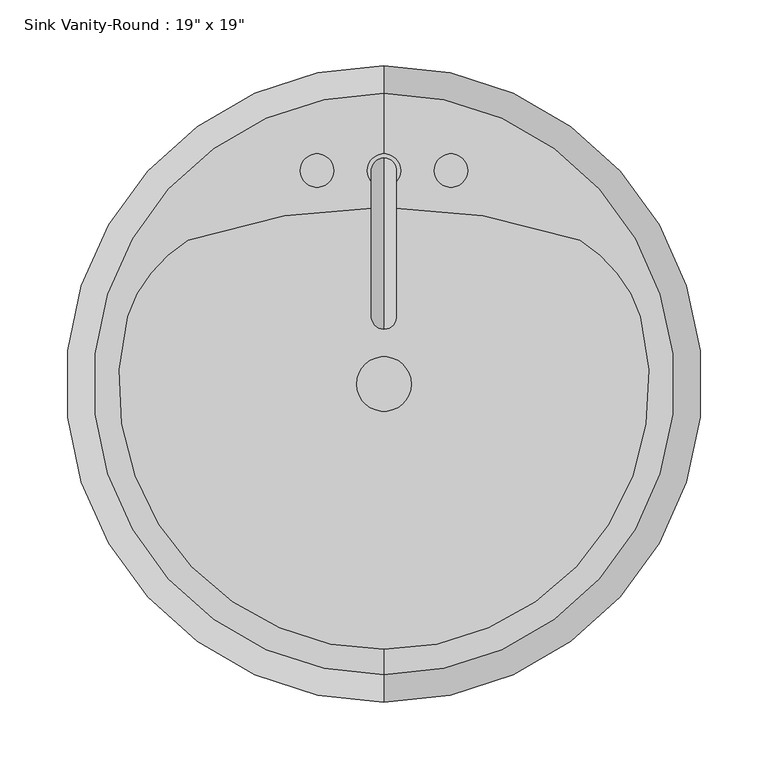
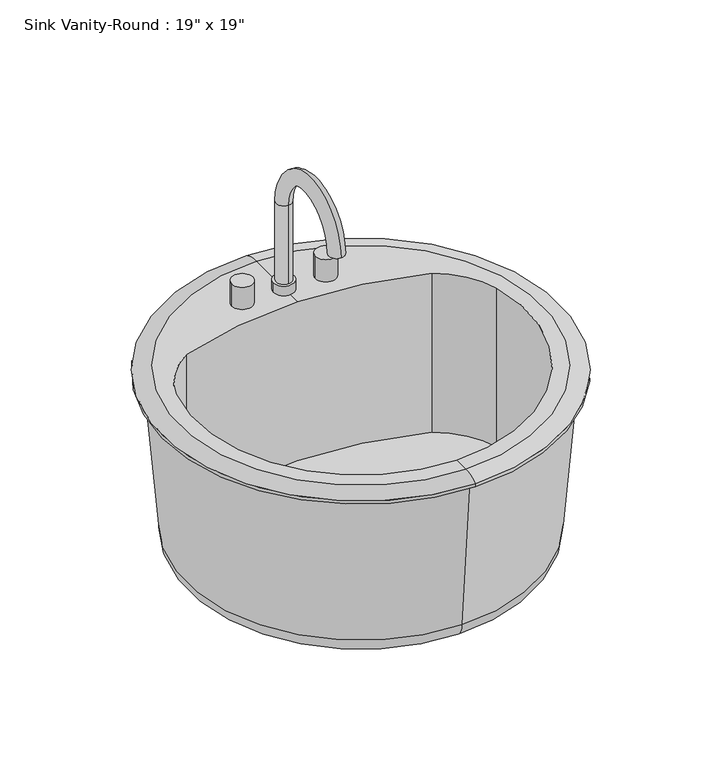
"""IFC4 building model written with IfcOpenShell, lengths in millimetres: flow terminal geometry."""

import ifcopenshell
import ifcopenshell.guid

model = None  # the IFC model being written
_history = None  # IfcOwnerHistory: only IFC2X3 demands one
_inside = {}  # id of a spatial element -> (the spatial element, [elements in it])
_under = {}  # id of a project, library or spatial element -> (it, [spatial elements below it])
_declared = {}  # id of a project -> (the project, [libraries it declares])
_typed = {}  # id of a type object -> (the type object, [elements of that type])
_made_of = {}  # id of a material, layer set ... -> (it, [elements and type objects made of it])


def new_model(schema):
    """Start an empty IFC model of exactly this schema.

    Asked for "IFC4X3", IfcOpenShell would pick the latest addendum, in which some entities
    have other attributes; the version numbers below select the first issue.
    IFC2X3 requires an IfcOwnerHistory on every rooted entity: one is made here for all.
    """
    global model, _history
    if schema == "IFC4X3":
        model = ifcopenshell.file(schema_version=(4, 3, 0, 0))
    else:
        model = ifcopenshell.file(schema=schema)
    _inside.clear()
    _under.clear()
    _declared.clear()
    _typed.clear()
    _made_of.clear()
    _history = None
    if model.schema == "IFC2X3":
        org = make("IfcOrganization", Name="unknown")
        user = make(
            "IfcPersonAndOrganization",
            ThePerson=make("IfcPerson", FamilyName="unknown"),
            TheOrganization=org,
        )
        app = make(
            "IfcApplication",
            ApplicationDeveloper=org,
            Version="unknown",
            ApplicationFullName="unknown",
            ApplicationIdentifier="unknown",
        )
        _history = make(
            "IfcOwnerHistory",
            OwningUser=user,
            OwningApplication=app,
            ChangeAction="ADDED",
            CreationDate=0,
        )
    return model


def make(cls, **values):
    """One entity of the class cls with the attributes given. An attribute that is None is left unset."""
    return model.create_entity(
        cls, **{name: value for name, value in values.items() if value is not None}
    )


def rooted(cls, **values):
    """An entity with a GlobalId (a new one), such as an element, a storey or a relation."""
    return make(cls, GlobalId=ifcopenshell.guid.new(), OwnerHistory=_history, **values)


def si_unit(unit_type, name, prefix=None):
    """IfcSIUnit, for example si_unit("LENGTHUNIT", "METRE", prefix="MILLI")."""
    return make("IfcSIUnit", UnitType=unit_type, Prefix=prefix, Name=name)


def assignment(units):
    """IfcUnitAssignment: the units of a project."""
    return None if units is None else make("IfcUnitAssignment", Units=units)


def point(xyz):
    """IfcCartesianPoint."""
    return None if xyz is None else make("IfcCartesianPoint", Coordinates=xyz)


def direction(xyz):
    """IfcDirection."""
    return None if xyz is None else make("IfcDirection", DirectionRatios=xyz)


def frame(location, z_axis=None, x_axis=None):
    """IfcAxis2Placement3D, a coordinate frame: its origin and axes. An axis left out is left unset."""
    return make(
        "IfcAxis2Placement3D",
        Location=point(location),
        Axis=direction(z_axis),
        RefDirection=direction(x_axis),
    )


def frame_2d(location, x_axis=None):
    """IfcAxis2Placement2D, a coordinate frame in the plane: its origin and x axis."""
    return make(
        "IfcAxis2Placement2D", Location=point(location), RefDirection=direction(x_axis)
    )


def origin():
    """The frame at (0, 0, 0) with its axes left unset."""
    return frame((0.0, 0.0, 0.0))


def place(relative_to, where):
    """IfcLocalPlacement: puts the frame where relative to a parent placement (None: the world)."""
    return make(
        "IfcLocalPlacement", PlacementRelTo=relative_to, RelativePlacement=where
    )


def context(
    kind, dimensions, precision=None, world=None, true_north=None, identifier=None
):
    """IfcGeometricRepresentationContext, for example the 3D "Model" context."""
    return make(
        "IfcGeometricRepresentationContext",
        ContextIdentifier=identifier,
        ContextType=kind,
        CoordinateSpaceDimension=dimensions,
        Precision=precision,
        WorldCoordinateSystem=world,
        TrueNorth=true_north,
    )


def project(units=None, contexts=None):
    """IfcProject with its units and contexts."""
    return rooted(
        "IfcProject",
        Name="project",
        RepresentationContexts=contexts,
        UnitsInContext=assignment(units),
    )


def spatial(cls, under=None, at=None, **own):
    """A site, building, storey or space (cls), placed at a placement, below another one or the project."""
    s = rooted(cls, ObjectPlacement=at, **own)
    if under is not None:
        _under.setdefault(under.id(), (under, []))[1].append(s)
    return s


def polyline(points):
    """IfcPolyline through the points."""
    return make("IfcPolyline", Points=[point(p) for p in points])


def circle_curve(where, radius):
    """IfcCircle in the frame where."""
    return make("IfcCircle", Position=where, Radius=radius)


def ellipse_curve(where, semi_axis1, semi_axis2):
    """IfcEllipse in the frame where."""
    return make(
        "IfcEllipse", Position=where, SemiAxis1=semi_axis1, SemiAxis2=semi_axis2
    )


def trimmed(basis, trim1, trim2, sense, master):
    """IfcTrimmedCurve: the piece of a basis curve between two trims."""
    return make(
        "IfcTrimmedCurve",
        BasisCurve=basis,
        Trim1=trim1,
        Trim2=trim2,
        SenseAgreement=sense,
        MasterRepresentation=master,
    )


def segment(curve, same_sense, transition):
    """IfcCompositeCurveSegment."""
    return make(
        "IfcCompositeCurveSegment",
        Transition=transition,
        SameSense=same_sense,
        ParentCurve=curve,
    )


def composite_curve(segments, self_intersect=None):
    """IfcCompositeCurve: segments joined end to end."""
    return make("IfcCompositeCurve", Segments=segments, SelfIntersect=self_intersect)


def outline(outer, holes=None, kind="AREA"):
    """IfcArbitraryClosedProfileDef: a profile drawn as a closed curve; with holes, ...WithVoids."""
    if holes is None:
        return make("IfcArbitraryClosedProfileDef", ProfileType=kind, OuterCurve=outer)
    return make(
        "IfcArbitraryProfileDefWithVoids",
        ProfileType=kind,
        OuterCurve=outer,
        InnerCurves=holes,
    )


def extrude(swept, where, along, depth):
    """IfcExtrudedAreaSolid: the profile swept, set in the frame where, extruded along a direction by depth."""
    return make(
        "IfcExtrudedAreaSolid",
        SweptArea=swept,
        Position=where,
        ExtrudedDirection=direction(along),
        Depth=depth,
    )


def shape(context_of_items, identifier, shape_type, items):
    """IfcShapeRepresentation: the items that make up one representation, for example the "Body"."""
    return make(
        "IfcShapeRepresentation",
        ContextOfItems=context_of_items,
        RepresentationIdentifier=identifier,
        RepresentationType=shape_type,
        Items=items,
    )


def source(mapping_origin, context_of_items, identifier, shape_type, items):
    """IfcRepresentationMap: a shape defined once, which mapped items show again and again."""
    return make(
        "IfcRepresentationMap",
        MappingOrigin=mapping_origin,
        MappedRepresentation=shape(context_of_items, identifier, shape_type, items),
    )


def transform(
    local_origin,
    x_axis=None,
    y_axis=None,
    z_axis=None,
    scale=None,
    scale2=None,
    scale3=None,
    uniform=True,
):
    """IfcCartesianTransformationOperator3D, or its non-uniform kind. x_axis, y_axis, z_axis: its Axis1, 2, 3."""
    if uniform:
        return make(
            "IfcCartesianTransformationOperator3D",
            Axis1=direction(x_axis),
            Axis2=direction(y_axis),
            LocalOrigin=point(local_origin),
            Scale=scale,
            Axis3=direction(z_axis),
        )
    return make(
        "IfcCartesianTransformationOperator3DnonUniform",
        Axis1=direction(x_axis),
        Axis2=direction(y_axis),
        LocalOrigin=point(local_origin),
        Scale=scale,
        Axis3=direction(z_axis),
        Scale2=scale2,
        Scale3=scale3,
    )


def mapped(mapping_source, mapping_target):
    """IfcMappedItem: shows the shape of a source again, moved by a transform."""
    return make(
        "IfcMappedItem", MappingSource=mapping_source, MappingTarget=mapping_target
    )


def made_of(thing, what):
    """Note that an element or type object is made of a material, layer set ...; save() writes the relation."""
    if what is not None:
        _made_of.setdefault(what.id(), (what, []))[1].append(thing)
    return thing


def element(
    cls,
    number,
    at=None,
    inside=None,
    cuts=None,
    type_object=None,
    material=None,
    context=None,
    identifier="Body",
    shape_type=None,
    held_by="IfcProductDefinitionShape",
    body=None,
    shapes=None,
    **own,
):
    """One element of the class cls, such as IfcWall. Its Tag is "e" and its number.

    at: its placement. inside: the storey or other place that contains it. cuts: it is an
    opening in that element (IfcRelVoidsElement). A single representation is given by context,
    identifier, shape_type and body (its items); several are given by shapes. held_by: the class
    of the entity that holds the representations. save() writes the other relations.
    """
    e = rooted(cls, Tag="e%d" % number, ObjectPlacement=at, **own)
    if body is not None:
        shapes = [shape(context, identifier, shape_type, body)]
    if shapes is not None:
        e.Representation = make(held_by, Representations=shapes)
    if inside is not None:
        _inside.setdefault(inside.id(), (inside, []))[1].append(e)
    if cuts is not None:
        rooted(
            "IfcRelVoidsElement", RelatingBuildingElement=cuts, RelatedOpeningElement=e
        )
    if type_object is not None:
        _typed.setdefault(type_object.id(), (type_object, []))[1].append(e)
    return made_of(e, material)


def aggregate(whole, parts):
    """IfcRelAggregates: a whole, such as a stair, and the parts it consists of."""
    return rooted("IfcRelAggregates", RelatingObject=whole, RelatedObjects=parts)


def save(model, path):
    """Write the relations noted so far, then the file.

    IfcRelAggregates (storeys below a building ...), IfcRelContainedInSpatialStructure (elements
    in a storey), IfcRelDefinesByType, IfcRelAssociatesMaterial and IfcRelDeclares: one each for
    every whole, place, type object, material and project.
    """
    for whole, parts in _under.values():
        aggregate(whole, parts)
    for where, things in _inside.values():
        rooted(
            "IfcRelContainedInSpatialStructure",
            RelatedElements=things,
            RelatingStructure=where,
        )
    for kind, things in _typed.values():
        rooted("IfcRelDefinesByType", RelatedObjects=things, RelatingType=kind)
    for what, things in _made_of.values():
        rooted("IfcRelAssociatesMaterial", RelatedObjects=things, RelatingMaterial=what)
    for by, libraries in _declared.values():
        rooted("IfcRelDeclares", RelatingContext=by, RelatedDefinitions=libraries)
    model.write(path)


def plane_surface(at):
    """IfcPlane: the flat surface through the origin of the frame at, square to its z axis."""
    return make("IfcPlane", Position=at)


def cylinder_surface(at, radius):
    """IfcCylindricalSurface: all points at the distance radius from the z axis of the frame at."""
    return make("IfcCylindricalSurface", Position=at, Radius=radius)


def revolved_surface(curve, axis_point, axis_direction):
    """IfcSurfaceOfRevolution: the curve turned about the line through axis_point along axis_direction."""
    return make(
        "IfcSurfaceOfRevolution",
        SweptCurve=make("IfcArbitraryOpenProfileDef", ProfileType="CURVE", Curve=curve),
        AxisPosition=make("IfcAxis1Placement", Location=point(axis_point), Axis=direction(axis_direction)),
    )


def advanced_brep(points, edges, surfaces, faces):
    """IfcAdvancedBrep: a solid bounded by faces that lie on surfaces and meet in shared edges.

    An edge is (start, end): straight between two places in points (the first is 0);
    or (start, end, curve); or (start, end, curve, False) where it runs against its curve.
    A face is (place in surfaces, loops), or (place, loops, False) where it looks against
    its surface's normal. A loop lists edges by number (the first is 1), with a minus sign
    where the edge is run from its end to its start. The first loop is the outer one.
    """
    corners = [point(p) for p in points]
    vertices = [make("IfcVertexPoint", VertexGeometry=c) for c in corners]
    made = []
    for start, end, *more in edges:
        made.append(
            make(
                "IfcEdgeCurve",
                EdgeStart=vertices[start],
                EdgeEnd=vertices[end],
                EdgeGeometry=more[0] if more else make("IfcPolyline", Points=[corners[start], corners[end]]),
                SameSense=more[1] if len(more) > 1 else True,
            )
        )
    hull = []
    for where, loops, *sense in faces:
        bounds = []
        for j, loop in enumerate(loops):
            ring = [make("IfcOrientedEdge", EdgeElement=made[abs(k) - 1], Orientation=k > 0) for k in loop]
            bounds.append(
                make(
                    "IfcFaceOuterBound" if j == 0 else "IfcFaceBound",
                    Bound=make("IfcEdgeLoop", EdgeList=ring),
                    Orientation=True,
                )
            )
        hull.append(make("IfcAdvancedFace", Bounds=bounds, FaceSurface=surfaces[where], SameSense=sense[0] if sense else True))
    return make("IfcAdvancedBrep", Outer=make("IfcClosedShell", CfsFaces=hull))


def flow_terminal_d49f872f(model_context):
    return source(origin(), model_context, "Body", "SolidModel", [
        advanced_brep(
        [(83.9517406, 247.0927185, 796.925), (109.3517406, 247.0927185, 796.925), (96.6517406, 237.5677185, 909.6375), (96.6517406, 256.6177185, 909.6375), (96.6517406, 256.6177185, 809.1602909), (96.6517406, 237.5677185, 809.1602909), (96.6517406, 145.7775038, 909.6375), (96.6517406, 126.7275038, 909.6375), (83.9517406, 247.0927185, 809.1602909), (109.3517406, 247.0927185, 809.1602909)],
        [
            (0, 1, circle_curve(frame((96.6517406, 247.0927185, 796.925), z_axis=(0.0, 0.0, -1.0), x_axis=(1.0, 0.0, 0.0)), 12.7)),
            (1, 0, circle_curve(frame((96.6517406, 247.0927185, 796.925), z_axis=(0.0, 0.0, -1.0), x_axis=(1.0, 0.0, 0.0)), 12.7)),
            (2, 3, circle_curve(frame((96.6517406, 247.0927185, 909.6375), z_axis=(0.0, 0.0, -1.0), x_axis=(0.0, 1.0, 0.0)), 9.525)),
            (3, 4),
            (4, 5, circle_curve(frame((96.6517406, 247.0927185, 809.1602909), z_axis=(0.0, 0.0, 1.0), x_axis=(0.0, 1.0, 0.0)), 9.525)),
            (5, 2),
            (3, 2, circle_curve(frame((96.6517406, 247.0927185, 909.6375), z_axis=(0.0, 0.0, -1.0), x_axis=(0.0, 1.0, 0.0)), 9.525)),
            (5, 4, circle_curve(frame((96.6517406, 247.0927185, 809.1602909), z_axis=(0.0, 0.0, 1.0), x_axis=(0.0, 1.0, 0.0)), 9.525)),
            (6, 7, circle_curve(frame((96.6517406, 136.2525038, 909.6375), z_axis=(0.0, 0.0, -1.0), x_axis=(0.0, -1.0, 0.0)), 9.525)),
            (7, 6, circle_curve(frame((96.6517406, 136.2525038, 909.6375), z_axis=(0.0, 0.0, -1.0), x_axis=(0.0, -1.0, 0.0)), 9.525)),
            (2, 6, circle_curve(frame((96.6517406, 191.6726112, 909.6375), z_axis=(1.0, 0.0, 0.0), x_axis=(0.0, 1.0, 0.0)), 45.8951073)),
            (7, 3, circle_curve(frame((96.6517406, 191.6726112, 909.6375), z_axis=(-1.0, 0.0, 0.0), x_axis=(0.0, 1.0, 0.0)), 64.9451073)),
            (8, 9, circle_curve(frame((96.6517406, 247.0927185, 809.1602909), z_axis=(0.0, 0.0, 1.0), x_axis=(1.0, 0.0, 0.0)), 12.7)),
            (9, 8, circle_curve(frame((96.6517406, 247.0927185, 809.1602909), z_axis=(0.0, 0.0, 1.0), x_axis=(1.0, 0.0, 0.0)), 12.7)),
            (8, 0),
            (1, 9),
        ],
        [
            plane_surface(frame((96.6517406, 237.5677185, 796.925), z_axis=(0.0, 0.0, -1.0), x_axis=(1.0, 0.0, 0.0))),
            cylinder_surface(frame((96.6517406, 247.0927185, 796.925), z_axis=(0.0, 0.0, -1.0), x_axis=(0.0, 1.0, 0.0)), 9.525),
            plane_surface(frame((96.6517406, 191.6726112, 909.6375), z_axis=(0.0, 0.0, -1.0), x_axis=(0.0, -1.0, 0.0))),
            revolved_surface(trimmed(ellipse_curve(frame((96.6517406, 247.0927185, 909.6375), z_axis=(0.0, 0.0, -1.0), x_axis=(0.0, 1.0, 0.0)), 9.525, 9.525), [point((96.6517406, 237.5677185, 909.6375))], [point((96.6517406, 256.6177185, 909.6375))], True, "CARTESIAN"), (96.6517406, 191.6726112, 909.6375), (1.0, 0.0, 0.0)),
            revolved_surface(trimmed(ellipse_curve(frame((96.6517406, 247.0927185, 909.6375), z_axis=(0.0, 0.0, -1.0), x_axis=(0.0, 1.0, 0.0)), 9.525, 9.525), [point((96.6517406, 256.6177185, 909.6375))], [point((96.6517406, 237.5677185, 909.6375))], True, "CARTESIAN"), (96.6517406, 191.6726112, 909.6375), (1.0, 0.0, 0.0)),
            plane_surface(frame((109.3517406, 247.0927185, 809.1602909), z_axis=(0.0, 0.0, 1.0), x_axis=(0.0, 1.0, 0.0))),
            cylinder_surface(frame((96.6517406, 247.0927185, 796.925), z_axis=(0.0, 0.0, 1.0), x_axis=(1.0, 0.0, 0.0)), 12.7),
        ],
        [
            (0, [[1, 2]]),
            (1, [[3, 4, 5, 6]]),
            (1, [[7, -6, 8, -4]]),
            (2, [[9, 10]]),
            (3, [[-3, 11, -10, 12]]),
            (4, [[-7, -12, -9, -11]]),
            (5, [[13, 14], [-5, -8]]),
            (6, [[-13, 15, -2, 16]]),
            (6, [[-14, -16, -1, -15]]),
        ],
    ),
        extrude(outline(composite_curve([segment(trimmed(circle_curve(frame_2d((45.8517406, 247.0927185)), 12.7), [point((33.1517406, 247.0927185))], [point((58.5517406, 247.0927185))], False, "CARTESIAN"), True, "CONTINUOUS"), segment(trimmed(circle_curve(frame_2d((45.8517406, 247.0927185)), 12.7), [point((58.5517406, 247.0927185))], [point((33.1517406, 247.0927185))], False, "CARTESIAN"), True, "CONTINUOUS")], self_intersect=False)), frame((0.0, 0.0, 796.925), z_axis=(0.0, 0.0, 1.0), x_axis=(1.0, 0.0, 0.0)), (0.0, 0.0, 1.0), 28.575),
        extrude(outline(composite_curve([segment(trimmed(circle_curve(frame_2d((147.4517406, 247.0927185)), 12.7), [point((134.7517406, 247.0927185))], [point((160.1517406, 247.0927185))], False, "CARTESIAN"), True, "CONTINUOUS"), segment(trimmed(circle_curve(frame_2d((147.4517406, 247.0927185)), 12.7), [point((160.1517406, 247.0927185))], [point((134.7517406, 247.0927185))], False, "CARTESIAN"), True, "CONTINUOUS")], self_intersect=False)), frame((0.0, 0.0, 796.925), z_axis=(0.0, 0.0, 1.0), x_axis=(1.0, 0.0, 0.0)), (0.0, 0.0, 1.0), 28.575),
        extrude(outline(composite_curve([segment(trimmed(circle_curve(frame_2d((96.6517406, 85.1677185)), 20.6375), [point((76.0142406, 85.1677185))], [point((117.2892406, 85.1677185))], False, "CARTESIAN"), True, "CONTINUOUS"), segment(trimmed(circle_curve(frame_2d((96.6517406, 85.1677185)), 20.6375), [point((117.2892406, 85.1677185))], [point((76.0142406, 85.1677185))], False, "CARTESIAN"), True, "CONTINUOUS")], self_intersect=False)), frame((0.0, 0.0, 571.5), z_axis=(0.0, 0.0, 1.0), x_axis=(1.0, 0.0, 0.0)), (0.0, 0.0, 1.0), 21.1842611),
        advanced_brep(
        [(96.6517406, -135.3870093, 796.925), (96.6517406, 305.7224463, 796.925), (96.6517406, 326.4677185, 791.36875), (96.6517406, -156.1322815, 791.36875), (96.6517406, -116.2405705, 796.925), (-98.1703414, 136.2525038, 796.925), (-52.1534933, 194.0861398, 796.925), (96.6517406, 219.2662048, 796.925), (245.4569744, 194.0861398, 796.925), (291.4738225, 136.2525038, 796.925), (96.6517406, -107.1264028, 571.5), (96.6517406, 277.4618398, 571.5), (96.6517406, 85.1677185, 571.5), (96.6517406, -127.6827361, 592.6842611), (96.6517406, 298.0181731, 592.6842611), (96.6517406, -144.2260315, 787.4), (96.6517406, 314.5614685, 787.4), (96.6517406, -156.1322815, 787.4), (96.6517406, 326.4677185, 787.4), (245.4569744, 194.0861398, 592.6842611), (-52.1534933, 194.0861398, 592.6842611), (-98.1703414, 136.2525038, 592.6842611), (291.4738225, 136.2525038, 592.6842611)],
        [
            (0, 1, circle_curve(frame((96.6517406, 85.1677185, 796.925), z_axis=(0.0, 0.0, -1.0), x_axis=(0.0, 1.0, 0.0)), 220.5547278)),
            (1, 2, circle_curve(frame((96.6517406, 309.4374616, 769.289434), z_axis=(-1.0, 0.0, 0.0), x_axis=(0.0, 1.0, 0.0)), 27.8841505)),
            (2, 3, circle_curve(frame((96.6517406, 85.1677185, 791.36875), z_axis=(0.0, 0.0, 1.0), x_axis=(0.0, 1.0, 0.0)), 241.3)),
            (3, 0, circle_curve(frame((96.6517406, -139.1020246, 769.289434), z_axis=(-1.0, 0.0, 0.0), x_axis=(0.0, -1.0, 0.0)), 27.8841505)),
            (1, 0, circle_curve(frame((96.6517406, 85.1677185, 796.925), z_axis=(0.0, 0.0, -1.0), x_axis=(0.0, 1.0, 0.0)), 220.5547278)),
            (3, 2, circle_curve(frame((96.6517406, 85.1677185, 791.36875), z_axis=(0.0, 0.0, 1.0), x_axis=(0.0, 1.0, 0.0)), 241.3)),
            (0, 4),
            (4, 5, circle_curve(frame((96.6517406, 85.1677185, 796.925), z_axis=(0.0, 0.0, -1.0), x_axis=(1.0, 0.0, 0.0)), 201.408289)),
            (5, 6, circle_curve(frame((1.3689689, 104.2755165, 796.925), z_axis=(0.0, 0.0, -1.0), x_axis=(1.0, 0.0, 0.0)), 104.5495194)),
            (6, 7, circle_curve(frame((96.6517406, -233.0168462, 796.925), z_axis=(0.0, 0.0, -1.0), x_axis=(1.0, 0.0, 0.0)), 452.283051)),
            (7, 1),
            (7, 8, circle_curve(frame((96.6517406, -233.0168462, 796.925), z_axis=(0.0, 0.0, -1.0), x_axis=(1.0, 0.0, 0.0)), 452.283051)),
            (8, 9, circle_curve(frame((191.9345122, 104.2755165, 796.925), z_axis=(0.0, 0.0, -1.0), x_axis=(1.0, 0.0, 0.0)), 104.5495194)),
            (9, 4, circle_curve(frame((96.6517406, 85.1677185, 796.925), z_axis=(0.0, 0.0, -1.0), x_axis=(1.0, 0.0, 0.0)), 201.408289)),
            (10, 11, circle_curve(frame((96.6517406, 85.1677185, 571.5), z_axis=(0.0, 0.0, -1.0), x_axis=(0.0, 1.0, 0.0)), 192.2941213)),
            (11, 12),
            (12, 10),
            (11, 10, circle_curve(frame((96.6517406, 85.1677185, 571.5), z_axis=(0.0, 0.0, -1.0), x_axis=(0.0, 1.0, 0.0)), 192.2941213)),
            (10, 13, circle_curve(frame((96.6517406, -107.1264028, 592.0656396), z_axis=(-1.0, 0.0, 0.0), x_axis=(0.0, -1.0, 0.0)), 20.5656396)),
            (13, 14, circle_curve(frame((96.6517406, 85.1677185, 592.6842611), z_axis=(0.0, 0.0, -1.0), x_axis=(0.0, 1.0, 0.0)), 212.8504546)),
            (14, 11, circle_curve(frame((96.6517406, 277.4618398, 592.0656396), z_axis=(-1.0, 0.0, 0.0), x_axis=(0.0, 1.0, 0.0)), 20.5656396)),
            (14, 13, circle_curve(frame((96.6517406, 85.1677185, 592.6842611), z_axis=(0.0, 0.0, -1.0), x_axis=(0.0, 1.0, 0.0)), 212.8504546)),
            (13, 15),
            (15, 16, circle_curve(frame((96.6517406, 85.1677185, 787.4), z_axis=(0.0, 0.0, -1.0), x_axis=(0.0, 1.0, 0.0)), 229.39375)),
            (16, 14),
            (16, 15, circle_curve(frame((96.6517406, 85.1677185, 787.4), z_axis=(0.0, 0.0, -1.0), x_axis=(0.0, 1.0, 0.0)), 229.39375)),
            (15, 17),
            (17, 18, circle_curve(frame((96.6517406, 85.1677185, 787.4), z_axis=(0.0, 0.0, -1.0), x_axis=(0.0, 1.0, 0.0)), 241.3)),
            (18, 16),
            (18, 17, circle_curve(frame((96.6517406, 85.1677185, 787.4), z_axis=(0.0, 0.0, -1.0), x_axis=(0.0, 1.0, 0.0)), 241.3)),
            (2, 18),
            (17, 3),
            (19, 20, circle_curve(frame((96.6517406, -233.0168462, 592.6842611), z_axis=(0.0, 0.0, 1.0), x_axis=(1.0, 0.0, 0.0)), 452.283051)),
            (20, 21, circle_curve(frame((1.3689689, 104.2755165, 592.6842611), z_axis=(0.0, 0.0, 1.0), x_axis=(1.0, 0.0, 0.0)), 104.5495194)),
            (21, 22, circle_curve(frame((96.6517406, 85.1677185, 592.6842611), z_axis=(0.0, 0.0, 1.0), x_axis=(1.0, 0.0, 0.0)), 201.408289)),
            (22, 19, circle_curve(frame((191.9345122, 104.2755165, 592.6842611), z_axis=(0.0, 0.0, 1.0), x_axis=(1.0, 0.0, 0.0)), 104.5495194)),
            (19, 8),
            (6, 20),
            (5, 21),
            (9, 22),
        ],
        [
            revolved_surface(trimmed(ellipse_curve(frame((96.6517406, 309.4374616, 769.289434), z_axis=(1.0, 0.0, 0.0), x_axis=(0.0, 1.0, 0.0)), 27.8841505, 27.8841505), [point((96.6517406, 326.4677185, 791.36875))], [point((96.6517406, 305.7224463, 796.925))], True, "CARTESIAN"), (96.6517406, 85.1677185, 796.925), (0.0, 0.0, 1.0)),
            plane_surface(frame((96.6517406, 85.1677185, 796.925), z_axis=(0.0, 0.0, 1.0), x_axis=(0.0, 1.0, 0.0))),
            plane_surface(frame((96.6517406, 85.1677185, 571.5), z_axis=(0.0, 0.0, -1.0), x_axis=(0.0, 1.0, 0.0))),
            revolved_surface(trimmed(ellipse_curve(frame((96.6517406, 277.4618398, 592.0656396), z_axis=(1.0, 0.0, 0.0), x_axis=(0.0, 1.0, 0.0)), 20.5656396, 20.5656396), [point((96.6517406, 277.4618398, 571.5))], [point((96.6517406, 298.0181731, 592.6842611))], True, "CARTESIAN"), (96.6517406, 85.1677185, 796.925), (0.0, 0.0, 1.0)),
            revolved_surface(polyline([(96.6517406, 298.0181731, 592.6842611), (96.6517406, 314.5614685, 787.4)]), (96.6517406, 85.1677185, 796.925), (0.0, 0.0, 1.0)),
            plane_surface(frame((96.6517406, 85.1677185, 787.4), z_axis=(0.0, 0.0, -1.0), x_axis=(0.0, 1.0, 0.0))),
            cylinder_surface(frame((96.6517406, 85.1677185, 796.925), z_axis=(0.0, 0.0, 1.0), x_axis=(0.0, 1.0, 0.0)), 241.3),
            plane_surface(frame((548.9347916, -233.0168462, 592.6842611), z_axis=(0.0, 0.0, 1.0), x_axis=(0.0, -1.0, 0.0))),
            revolved_surface(polyline([(548.9347916, -233.0168462, 796.925), (548.9347916, -233.0168462, 592.6842611)]), (96.6517406, -233.0168462, 592.6842611), (0.0, 0.0, 1.0)),
            revolved_surface(polyline([(105.91848829999999, 104.2755165, 796.925), (105.91848829999999, 104.2755165, 592.6842611)]), (1.3689689, 104.2755165, 592.6842611), (0.0, 0.0, 1.0)),
            revolved_surface(polyline([(298.0600296, 85.1677185, 796.925), (298.0600296, 85.1677185, 592.6842611)]), (96.6517406, 85.1677185, 592.6842611), (0.0, 0.0, 1.0)),
            revolved_surface(polyline([(296.4840316, 104.2755165, 796.925), (296.4840316, 104.2755165, 592.6842611)]), (191.9345122, 104.2755165, 592.6842611), (0.0, 0.0, 1.0)),
        ],
        [
            (0, [[1, 2, 3, 4]]),
            (0, [[-2, 5, -4, 6]]),
            (1, [[-1, 7, 8, 9, 10, 11]]),
            (1, [[-5, -11, 12, 13, 14, -7]]),
            (2, [[15, 16, 17]]),
            (2, [[-16, 18, -17]]),
            (3, [[-15, 19, 20, 21]]),
            (3, [[-18, -21, 22, -19]]),
            (4, [[-20, 23, 24, 25]]),
            (4, [[-22, -25, 26, -23]]),
            (5, [[-24, 27, 28, 29]]),
            (5, [[-26, -29, 30, -27]]),
            (6, [[-3, 31, -28, 32]]),
            (6, [[-6, -32, -30, -31]]),
            (7, [[33, 34, 35, 36]]),
            (8, [[-33, 37, -12, -10, 38]]),
            (9, [[-34, -38, -9, 39]]),
            (10, [[-35, -39, -8, -14, 40]]),
            (11, [[-36, -40, -13, -37]]),
        ],
    ),
    ])


if __name__ == "__main__":
    model = new_model("IFC4")
    model_context = context("Model", 3, world=origin())
    ifc_project = project(units=[si_unit("LENGTHUNIT", "METRE", prefix="MILLI")], contexts=[model_context])
    site = spatial("IfcSite", under=ifc_project)
    building = spatial("IfcBuilding", under=site)
    placement = place(None, origin())
    flow_terminal_shape = flow_terminal_d49f872f(model_context)
    element("IfcFlowTerminal", 1, ObjectType="Sink Vanity-Round : 19\" x 19\"", at=placement, inside=building, context=model_context, shape_type="MappedRepresentation", body=[
        mapped(flow_terminal_shape, transform((0.0, 0.0, 0.0), x_axis=(1.0, 0.0, 0.0), y_axis=(0.0, 1.0, 0.0), z_axis=(0.0, 0.0, 1.0))),
    ])
    save(model, "model.ifc")

# Revit data of these elements
# Type "Sink Vanity-Round : 19\" x 19\""
#   Assembly Code = "D2010400"
#   Top Of Counter = 2' - 7"
#   Basin Material = Porcelain, White
#   Faucet Material = Steel, Chrome Plated
#   Default Elevation = 0
# Element 1 (IfcFlowTerminal, "Sink Vanity-Round : 19\" x 19\"")
#   Materials on its faces: "Porcelain, White", "Steel, Chrome Plated"
# Materials
#   "Porcelain, White": class "Ceramic", colour RGB 244 244 244, transparency 0, Description = "Porcelain, ivory", Cost = 0
#   "Steel, Chrome Plated": class "Metal", colour RGB 120 120 120, transparency 0, Description = "Chromiuim plated steel", Cost = 0
